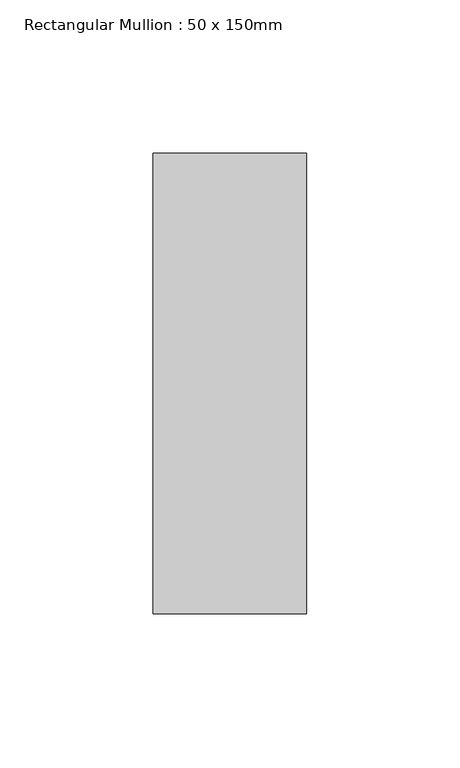
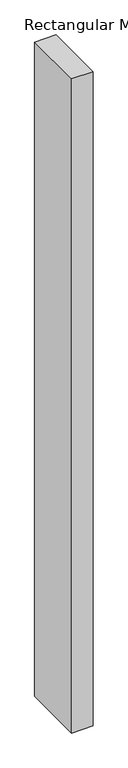
"""IFC4 building model written with IfcOpenShell, lengths in millimetres: member geometry, Rectangular Mullion : 50 x 150mm."""

from ifc_helpers import new_model, si_unit, frame, origin, place, context, project, spatial, polyline, outline, extrude, source, transform, mapped, element, save


def rectangular_mullion_50_x_150mm_f3b243f3(model_context):
    return source(origin(), model_context, "Body", "SweptSolid", [
        extrude(outline(polyline([(25.0, 75.0), (25.0, -75.0), (-25.0, -75.0), (-25.0, 75.0), (25.0, 75.0)])), frame((0.0, 0.0, -1615.0), z_axis=(0.0, 0.0, 1.0), x_axis=(1.0, 0.0, 0.0)), (0.0, 0.0, 1.0), 1615.0),
    ])


if __name__ == "__main__":
    model = new_model("IFC4")
    model_context = context("Model", 3, world=origin())
    ifc_project = project(units=[si_unit("LENGTHUNIT", "METRE", prefix="MILLI")], contexts=[model_context])
    site = spatial("IfcSite", under=ifc_project)
    building = spatial("IfcBuilding", under=site)
    placement = place(None, origin())
    rectangular_mullion_50_x_150mm_shape = rectangular_mullion_50_x_150mm_f3b243f3(model_context)
    element("IfcMember", 1, ObjectType="Rectangular Mullion : 50 x 150mm", at=placement, inside=building, context=model_context, shape_type="MappedRepresentation", body=[
        mapped(rectangular_mullion_50_x_150mm_shape, transform((0.0, 0.0, 0.0), x_axis=(1.0, 0.0, 0.0), y_axis=(0.0, 1.0, 0.0), z_axis=(0.0, 0.0, 1.0))),
    ])
    save(model, "model.ifc")

# Revit data of these elements
# Type "Rectangular Mullion : 50 x 150mm"
#   built-in parameter 1007304 = 0.492126 (stored number, unit not read)
#   built-in parameter 1007301 = 0.082021 (stored number, unit not read)
#   built-in parameter 1007300 = 0.082021 (stored number, unit not read)
# Element 1 (IfcMember, "Rectangular Mullion : 50 x 150mm")
#   Materials on its faces: "Metal - Aluminium"
# Materials
#   "Metal - Aluminium": class "Metal", colour RGB 247 247 247, transparency 0
